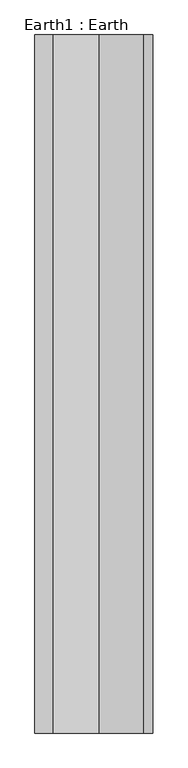
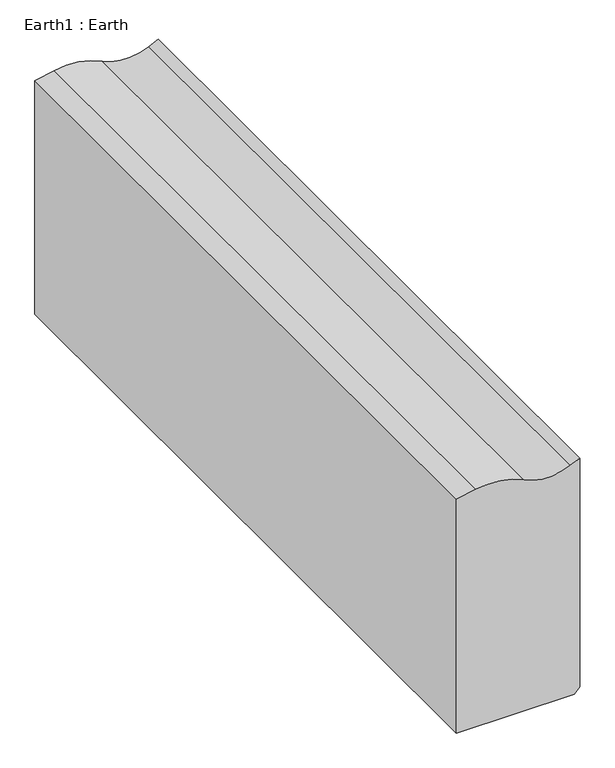
"""IFC4 building model written with IfcOpenShell, lengths in millimetres: proxy geometry, Earth1 : Earth."""

from ifc_helpers import new_model, si_unit, point, frame, frame_2d, origin, place, context, project, spatial, polyline, circle_curve, trimmed, segment, composite_curve, outline, extrude, source, transform, mapped, element, save


def earth1_earth_ca064f31(model_context):
    return source(origin(), model_context, "Body", "SweptSolid", [
        extrude(outline(composite_curve([segment(polyline([(32634.014262, -10045.4671386), (32634.014262, -9723.1517989), (32649.5954298, -9707.5706312), (33312.2775477, -9707.5706312), (33300.0908366, -9733.8927957)]), True, "CONTINUOUS"), segment(trimmed(circle_curve(frame_2d((33431.3167137, -9794.6481283)), 144.607888), [point((33300.0908366, -9733.8927957))], [point((33302.6181918, -9860.5884932))], True, "CARTESIAN"), True, "CONTINUOUS"), segment(trimmed(circle_curve(frame_2d((33120.1913863, -9954.0572443)), 204.9779178), [point((33302.6181918, -9860.5884932))], [point((33321.4784396, -9992.7802216))], False, "CARTESIAN"), True, "CONTINUOUS"), segment(polyline([(33321.4784396, -9992.7802216), (33311.3426943, -10045.4671386), (32634.014262, -10045.4671386)]), True, "CONTINUOUS")], self_intersect=False)), frame((0.0, 7182.1531721, 0.0), z_axis=(0.0, 1.0, 0.0), x_axis=(0.0, 0.0, 1.0)), (0.0, 0.0, 1.0), 2000.0),
    ])


if __name__ == "__main__":
    model = new_model("IFC4")
    model_context = context("Model", 3, world=origin())
    ifc_project = project(units=[si_unit("LENGTHUNIT", "METRE", prefix="MILLI")], contexts=[model_context])
    site = spatial("IfcSite", under=ifc_project)
    building = spatial("IfcBuilding", under=site)
    placement = place(None, origin())
    earth1_earth_shape = earth1_earth_ca064f31(model_context)
    element("IfcBuildingElementProxy", 1, Name="Earth1 : Earth", ObjectType="Earth1 : Earth", at=placement, inside=building, context=model_context, shape_type="MappedRepresentation", body=[
        mapped(earth1_earth_shape, transform((0.0, 0.0, 0.0), x_axis=(1.0, 0.0, 0.0), y_axis=(0.0, 1.0, 0.0), z_axis=(0.0, 0.0, 1.0))),
    ])
    save(model, "model.ifc")

# Revit data of these elements
# Type "Earth1 : Earth"
#   NameOverride = "Earth"
# Element 1 (IfcBuildingElementProxy, "Earth1 : Earth")
#   Materials on its faces: "GROUND SOIL"
# Materials
#   "GROUND SOIL": class "Unassigned", colour RGB 170 124 75, transparency 0, Cost = 0
